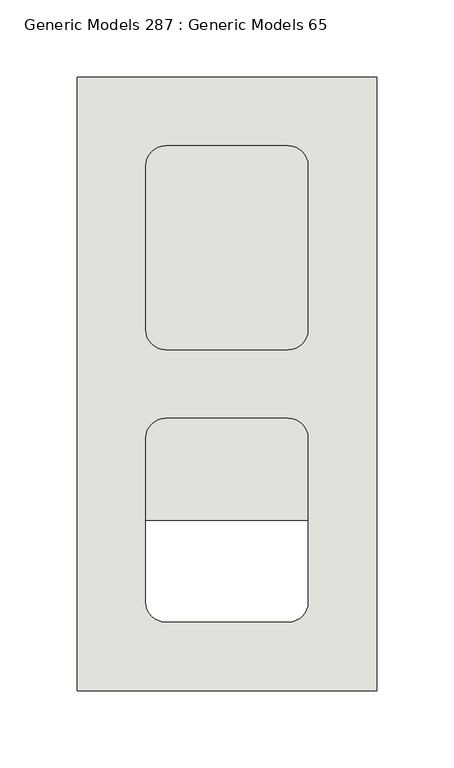
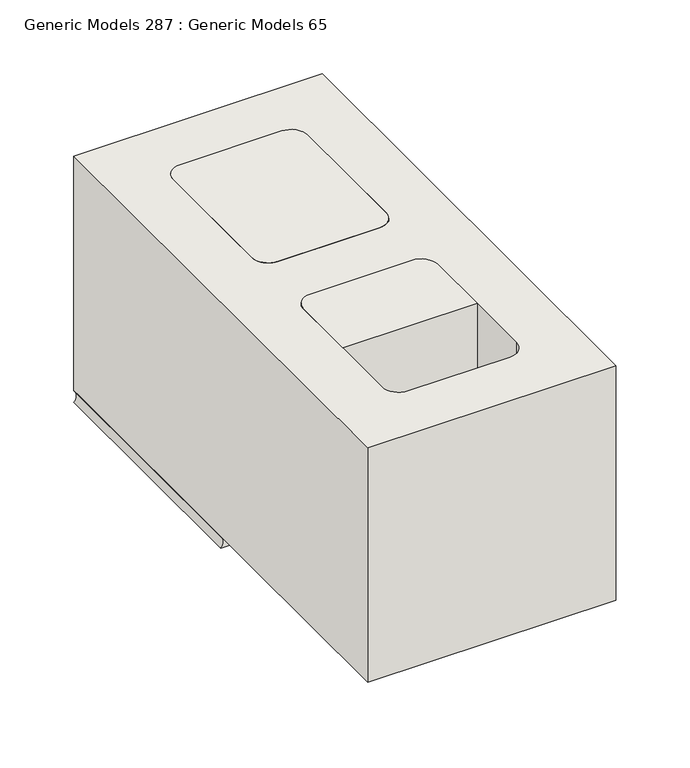
"""IFC4 building model written with IfcOpenShell, lengths in millimetres: wall geometry, Generic Models 287 : Generic Models 65."""

import ifcopenshell
import ifcopenshell.guid

model = None  # the IFC model being written
_history = None  # IfcOwnerHistory: only IFC2X3 demands one
_inside = {}  # id of a spatial element -> (the spatial element, [elements in it])
_under = {}  # id of a project, library or spatial element -> (it, [spatial elements below it])
_declared = {}  # id of a project -> (the project, [libraries it declares])
_typed = {}  # id of a type object -> (the type object, [elements of that type])
_made_of = {}  # id of a material, layer set ... -> (it, [elements and type objects made of it])


def new_model(schema):
    """Start an empty IFC model of exactly this schema.

    Asked for "IFC4X3", IfcOpenShell would pick the latest addendum, in which some entities
    have other attributes; the version numbers below select the first issue.
    IFC2X3 requires an IfcOwnerHistory on every rooted entity: one is made here for all.
    """
    global model, _history
    if schema == "IFC4X3":
        model = ifcopenshell.file(schema_version=(4, 3, 0, 0))
    else:
        model = ifcopenshell.file(schema=schema)
    _inside.clear()
    _under.clear()
    _declared.clear()
    _typed.clear()
    _made_of.clear()
    _history = None
    if model.schema == "IFC2X3":
        org = make("IfcOrganization", Name="unknown")
        user = make(
            "IfcPersonAndOrganization",
            ThePerson=make("IfcPerson", FamilyName="unknown"),
            TheOrganization=org,
        )
        app = make(
            "IfcApplication",
            ApplicationDeveloper=org,
            Version="unknown",
            ApplicationFullName="unknown",
            ApplicationIdentifier="unknown",
        )
        _history = make(
            "IfcOwnerHistory",
            OwningUser=user,
            OwningApplication=app,
            ChangeAction="ADDED",
            CreationDate=0,
        )
    return model


def make(cls, **values):
    """One entity of the class cls with the attributes given. An attribute that is None is left unset."""
    return model.create_entity(
        cls, **{name: value for name, value in values.items() if value is not None}
    )


def rooted(cls, **values):
    """An entity with a GlobalId (a new one), such as an element, a storey or a relation."""
    return make(cls, GlobalId=ifcopenshell.guid.new(), OwnerHistory=_history, **values)


def si_unit(unit_type, name, prefix=None):
    """IfcSIUnit, for example si_unit("LENGTHUNIT", "METRE", prefix="MILLI")."""
    return make("IfcSIUnit", UnitType=unit_type, Prefix=prefix, Name=name)


def assignment(units):
    """IfcUnitAssignment: the units of a project."""
    return None if units is None else make("IfcUnitAssignment", Units=units)


def point(xyz):
    """IfcCartesianPoint."""
    return None if xyz is None else make("IfcCartesianPoint", Coordinates=xyz)


def direction(xyz):
    """IfcDirection."""
    return None if xyz is None else make("IfcDirection", DirectionRatios=xyz)


def frame(location, z_axis=None, x_axis=None):
    """IfcAxis2Placement3D, a coordinate frame: its origin and axes. An axis left out is left unset."""
    return make(
        "IfcAxis2Placement3D",
        Location=point(location),
        Axis=direction(z_axis),
        RefDirection=direction(x_axis),
    )


def frame_2d(location, x_axis=None):
    """IfcAxis2Placement2D, a coordinate frame in the plane: its origin and x axis."""
    return make(
        "IfcAxis2Placement2D", Location=point(location), RefDirection=direction(x_axis)
    )


def origin():
    """The frame at (0, 0, 0) with its axes left unset."""
    return frame((0.0, 0.0, 0.0))


def origin_with_axes():
    """The frame at (0, 0, 0) with the z axis (0, 0, 1) and the x axis (1, 0, 0) written out."""
    return frame((0.0, 0.0, 0.0), z_axis=(0.0, 0.0, 1.0), x_axis=(1.0, 0.0, 0.0))


def place(relative_to, where):
    """IfcLocalPlacement: puts the frame where relative to a parent placement (None: the world)."""
    return make(
        "IfcLocalPlacement", PlacementRelTo=relative_to, RelativePlacement=where
    )


def context(
    kind, dimensions, precision=None, world=None, true_north=None, identifier=None
):
    """IfcGeometricRepresentationContext, for example the 3D "Model" context."""
    return make(
        "IfcGeometricRepresentationContext",
        ContextIdentifier=identifier,
        ContextType=kind,
        CoordinateSpaceDimension=dimensions,
        Precision=precision,
        WorldCoordinateSystem=world,
        TrueNorth=true_north,
    )


def project(units=None, contexts=None):
    """IfcProject with its units and contexts."""
    return rooted(
        "IfcProject",
        Name="project",
        RepresentationContexts=contexts,
        UnitsInContext=assignment(units),
    )


def spatial(cls, under=None, at=None, **own):
    """A site, building, storey or space (cls), placed at a placement, below another one or the project."""
    s = rooted(cls, ObjectPlacement=at, **own)
    if under is not None:
        _under.setdefault(under.id(), (under, []))[1].append(s)
    return s


def polyline(points):
    """IfcPolyline through the points."""
    return make("IfcPolyline", Points=[point(p) for p in points])


def circle_curve(where, radius):
    """IfcCircle in the frame where."""
    return make("IfcCircle", Position=where, Radius=radius)


def trimmed(basis, trim1, trim2, sense, master):
    """IfcTrimmedCurve: the piece of a basis curve between two trims."""
    return make(
        "IfcTrimmedCurve",
        BasisCurve=basis,
        Trim1=trim1,
        Trim2=trim2,
        SenseAgreement=sense,
        MasterRepresentation=master,
    )


def segment(curve, same_sense, transition):
    """IfcCompositeCurveSegment."""
    return make(
        "IfcCompositeCurveSegment",
        Transition=transition,
        SameSense=same_sense,
        ParentCurve=curve,
    )


def composite_curve(segments, self_intersect=None):
    """IfcCompositeCurve: segments joined end to end."""
    return make("IfcCompositeCurve", Segments=segments, SelfIntersect=self_intersect)


def outline(outer, holes=None, kind="AREA"):
    """IfcArbitraryClosedProfileDef: a profile drawn as a closed curve; with holes, ...WithVoids."""
    if holes is None:
        return make("IfcArbitraryClosedProfileDef", ProfileType=kind, OuterCurve=outer)
    return make(
        "IfcArbitraryProfileDefWithVoids",
        ProfileType=kind,
        OuterCurve=outer,
        InnerCurves=holes,
    )


def extrude(swept, where, along, depth):
    """IfcExtrudedAreaSolid: the profile swept, set in the frame where, extruded along a direction by depth."""
    return make(
        "IfcExtrudedAreaSolid",
        SweptArea=swept,
        Position=where,
        ExtrudedDirection=direction(along),
        Depth=depth,
    )


def shape(context_of_items, identifier, shape_type, items):
    """IfcShapeRepresentation: the items that make up one representation, for example the "Body"."""
    return make(
        "IfcShapeRepresentation",
        ContextOfItems=context_of_items,
        RepresentationIdentifier=identifier,
        RepresentationType=shape_type,
        Items=items,
    )


def source(mapping_origin, context_of_items, identifier, shape_type, items):
    """IfcRepresentationMap: a shape defined once, which mapped items show again and again."""
    return make(
        "IfcRepresentationMap",
        MappingOrigin=mapping_origin,
        MappedRepresentation=shape(context_of_items, identifier, shape_type, items),
    )


def transform(
    local_origin,
    x_axis=None,
    y_axis=None,
    z_axis=None,
    scale=None,
    scale2=None,
    scale3=None,
    uniform=True,
):
    """IfcCartesianTransformationOperator3D, or its non-uniform kind. x_axis, y_axis, z_axis: its Axis1, 2, 3."""
    if uniform:
        return make(
            "IfcCartesianTransformationOperator3D",
            Axis1=direction(x_axis),
            Axis2=direction(y_axis),
            LocalOrigin=point(local_origin),
            Scale=scale,
            Axis3=direction(z_axis),
        )
    return make(
        "IfcCartesianTransformationOperator3DnonUniform",
        Axis1=direction(x_axis),
        Axis2=direction(y_axis),
        LocalOrigin=point(local_origin),
        Scale=scale,
        Axis3=direction(z_axis),
        Scale2=scale2,
        Scale3=scale3,
    )


def mapped(mapping_source, mapping_target):
    """IfcMappedItem: shows the shape of a source again, moved by a transform."""
    return make(
        "IfcMappedItem", MappingSource=mapping_source, MappingTarget=mapping_target
    )


def made_of(thing, what):
    """Note that an element or type object is made of a material, layer set ...; save() writes the relation."""
    if what is not None:
        _made_of.setdefault(what.id(), (what, []))[1].append(thing)
    return thing


def element(
    cls,
    number,
    at=None,
    inside=None,
    cuts=None,
    type_object=None,
    material=None,
    context=None,
    identifier="Body",
    shape_type=None,
    held_by="IfcProductDefinitionShape",
    body=None,
    shapes=None,
    **own,
):
    """One element of the class cls, such as IfcWall. Its Tag is "e" and its number.

    at: its placement. inside: the storey or other place that contains it. cuts: it is an
    opening in that element (IfcRelVoidsElement). A single representation is given by context,
    identifier, shape_type and body (its items); several are given by shapes. held_by: the class
    of the entity that holds the representations. save() writes the other relations.
    """
    e = rooted(cls, Tag="e%d" % number, ObjectPlacement=at, **own)
    if body is not None:
        shapes = [shape(context, identifier, shape_type, body)]
    if shapes is not None:
        e.Representation = make(held_by, Representations=shapes)
    if inside is not None:
        _inside.setdefault(inside.id(), (inside, []))[1].append(e)
    if cuts is not None:
        rooted(
            "IfcRelVoidsElement", RelatingBuildingElement=cuts, RelatedOpeningElement=e
        )
    if type_object is not None:
        _typed.setdefault(type_object.id(), (type_object, []))[1].append(e)
    return made_of(e, material)


def aggregate(whole, parts):
    """IfcRelAggregates: a whole, such as a stair, and the parts it consists of."""
    return rooted("IfcRelAggregates", RelatingObject=whole, RelatedObjects=parts)


def save(model, path):
    """Write the relations noted so far, then the file.

    IfcRelAggregates (storeys below a building ...), IfcRelContainedInSpatialStructure (elements
    in a storey), IfcRelDefinesByType, IfcRelAssociatesMaterial and IfcRelDeclares: one each for
    every whole, place, type object, material and project.
    """
    for whole, parts in _under.values():
        aggregate(whole, parts)
    for where, things in _inside.values():
        rooted(
            "IfcRelContainedInSpatialStructure",
            RelatedElements=things,
            RelatingStructure=where,
        )
    for kind, things in _typed.values():
        rooted("IfcRelDefinesByType", RelatedObjects=things, RelatingType=kind)
    for what, things in _made_of.values():
        rooted("IfcRelAssociatesMaterial", RelatedObjects=things, RelatingMaterial=what)
    for by, libraries in _declared.values():
        rooted("IfcRelDeclares", RelatingContext=by, RelatedDefinitions=libraries)
    model.write(path)


def plane_surface(at):
    """IfcPlane: the flat surface through the origin of the frame at, square to its z axis."""
    return make("IfcPlane", Position=at)


def revolved_surface(curve, axis_point, axis_direction):
    """IfcSurfaceOfRevolution: the curve turned about the line through axis_point along axis_direction."""
    return make(
        "IfcSurfaceOfRevolution",
        SweptCurve=make("IfcArbitraryOpenProfileDef", ProfileType="CURVE", Curve=curve),
        AxisPosition=make("IfcAxis1Placement", Location=point(axis_point), Axis=direction(axis_direction)),
    )


def advanced_brep(points, edges, surfaces, faces):
    """IfcAdvancedBrep: a solid bounded by faces that lie on surfaces and meet in shared edges.

    An edge is (start, end): straight between two places in points (the first is 0);
    or (start, end, curve); or (start, end, curve, False) where it runs against its curve.
    A face is (place in surfaces, loops), or (place, loops, False) where it looks against
    its surface's normal. A loop lists edges by number (the first is 1), with a minus sign
    where the edge is run from its end to its start. The first loop is the outer one.
    """
    corners = [point(p) for p in points]
    vertices = [make("IfcVertexPoint", VertexGeometry=c) for c in corners]
    made = []
    for start, end, *more in edges:
        made.append(
            make(
                "IfcEdgeCurve",
                EdgeStart=vertices[start],
                EdgeEnd=vertices[end],
                EdgeGeometry=more[0] if more else make("IfcPolyline", Points=[corners[start], corners[end]]),
                SameSense=more[1] if len(more) > 1 else True,
            )
        )
    hull = []
    for where, loops, *sense in faces:
        bounds = []
        for j, loop in enumerate(loops):
            ring = [make("IfcOrientedEdge", EdgeElement=made[abs(k) - 1], Orientation=k > 0) for k in loop]
            bounds.append(
                make(
                    "IfcFaceOuterBound" if j == 0 else "IfcFaceBound",
                    Bound=make("IfcEdgeLoop", EdgeList=ring),
                    Orientation=True,
                )
            )
        hull.append(make("IfcAdvancedFace", Bounds=bounds, FaceSurface=surfaces[where], SameSense=sense[0] if sense else True))
    return make("IfcAdvancedBrep", Outer=make("IfcClosedShell", CfsFaces=hull))


def generic_models_287_generic_models_65_ef469ebf(model_context):
    return source(origin(), model_context, "Body", "SolidModel", [
        advanced_brep(
        [(430198.2125, 503.2375, 9.525), (430004.5375, 503.2375, 9.525), (430004.5375, 503.2375, 0.0), (430198.2125, 503.2375, 0.0), (430198.2125, 701.675, 9.525), (430198.2125, 701.675, 0.0), (430004.5375, 701.675, 0.0), (430004.5375, 701.675, 9.525), (430153.7625, 538.1625, 9.525), (430141.0625, 525.4625, 9.525), (430061.6875, 525.4625, 9.525), (430048.9875, 538.1625, 9.525), (430048.9875, 644.525, 9.525), (430061.6875, 657.225, 9.525), (430141.0625, 657.225, 9.525), (430153.7625, 644.525, 9.525), (430141.0625, 525.4625, 0.0), (430153.7625, 538.1625, 0.0), (430061.6875, 525.4625, 0.0), (430048.9875, 538.1625, 0.0), (430048.9875, 644.525, 0.0), (430061.6875, 657.225, 0.0), (430141.0625, 657.225, 0.0), (430153.7625, 644.525, 0.0)],
        [
            (0, 1),
            (1, 2, circle_curve(frame((429999.6545028, 503.2375, 4.7625), z_axis=(0.0, 1.0, 0.0), x_axis=(1.0, 0.0, 0.0)), 6.8209287)),
            (2, 3),
            (3, 0, circle_curve(frame((430203.0954972, 503.2375, 4.7625), z_axis=(0.0, 1.0, 0.0), x_axis=(-1.0, 0.0, 0.0)), 6.8209287)),
            (4, 5, circle_curve(frame((430203.0954972, 701.675, 4.7625), z_axis=(0.0, -1.0, 0.0), x_axis=(-1.0, 0.0, 0.0)), 6.8209287)),
            (5, 6),
            (6, 7, circle_curve(frame((429999.6545028, 701.675, 4.7625), z_axis=(0.0, -1.0, 0.0), x_axis=(1.0, 0.0, 0.0)), 6.8209287)),
            (7, 4),
            (0, 4),
            (7, 1),
            (8, 9, circle_curve(frame((430141.0625, 538.1625, 9.525), z_axis=(0.0, 0.0, -1.0), x_axis=(-1.0, 0.0, 0.0)), 12.7)),
            (9, 10),
            (10, 11, circle_curve(frame((430061.6875, 538.1625, 9.525), z_axis=(0.0, 0.0, -1.0), x_axis=(-1.0, 0.0, 0.0)), 12.7)),
            (11, 12),
            (12, 13, circle_curve(frame((430061.6875, 644.525, 9.525), z_axis=(0.0, 0.0, -1.0), x_axis=(-1.0, 0.0, 0.0)), 12.7)),
            (13, 14),
            (14, 15, circle_curve(frame((430141.0625, 644.525, 9.525), z_axis=(0.0, 0.0, -1.0), x_axis=(-1.0, 0.0, 0.0)), 12.7)),
            (15, 8),
            (16, 9),
            (8, 17),
            (17, 16, circle_curve(frame((430141.0625, 538.1625, 0.0), z_axis=(0.0, 0.0, -1.0), x_axis=(-1.0, 0.0, 0.0)), 12.7)),
            (16, 18),
            (18, 10),
            (18, 19, circle_curve(frame((430061.6875, 538.1625, 0.0), z_axis=(0.0, 0.0, -1.0), x_axis=(-1.0, 0.0, 0.0)), 12.7)),
            (19, 11),
            (19, 20),
            (20, 12),
            (20, 21, circle_curve(frame((430061.6875, 644.525, 0.0), z_axis=(0.0, 0.0, -1.0), x_axis=(-1.0, 0.0, 0.0)), 12.7)),
            (21, 13),
            (21, 22),
            (22, 14),
            (22, 23, circle_curve(frame((430141.0625, 644.525, 0.0), z_axis=(0.0, 0.0, -1.0), x_axis=(-1.0, 0.0, 0.0)), 12.7)),
            (23, 15),
            (23, 17),
            (6, 2),
            (5, 3),
        ],
        [
            plane_surface(frame((430101.375, 503.2375, 9.921875), z_axis=(0.0, -1.0, 0.0), x_axis=(0.0, 0.0, 1.0))),
            plane_surface(frame((430101.375, 701.675, 9.921875), z_axis=(0.0, 1.0, 0.0), x_axis=(0.0, 0.0, 1.0))),
            plane_surface(frame((430198.2125, 503.2375, 9.525), z_axis=(0.0, 0.0, 1.0), x_axis=(0.0, 1.0, 0.0))),
            revolved_surface(polyline([(430128.3625, 538.1625, 9.525000000000006), (430128.3625, 538.1625, 0.0)]), (430141.0625, 538.1625, 193.675), (0.0, 0.0, 1.0)),
            plane_surface(frame((430061.6875, 525.4625, 193.675), z_axis=(0.0, 1.0, 0.0), x_axis=(0.0, 0.0, -1.0))),
            revolved_surface(polyline([(430048.9875, 538.1625, 9.525000000000006), (430048.9875, 538.1625, 0.0)]), (430061.6875, 538.1625, 193.675), (0.0, 0.0, 1.0)),
            plane_surface(frame((430048.9875, 644.525, 193.675), z_axis=(1.0, 0.0, 0.0), x_axis=(0.0, 0.0, -1.0))),
            revolved_surface(polyline([(430048.9875, 644.525, 9.525000000000006), (430048.9875, 644.525, 0.0)]), (430061.6875, 644.525, 193.675), (0.0, 0.0, 1.0)),
            plane_surface(frame((430141.0625, 657.225, 193.675), z_axis=(0.0, -1.0, 0.0), x_axis=(0.0, 0.0, -1.0))),
            revolved_surface(polyline([(430128.3625, 644.525, 9.525000000000006), (430128.3625, 644.525, 0.0)]), (430141.0625, 644.525, 193.675), (0.0, 0.0, 1.0)),
            plane_surface(frame((430153.7625, 538.1625, 193.675), z_axis=(-1.0, 0.0, 0.0), x_axis=(0.0, 0.0, -1.0))),
            revolved_surface(polyline([(430006.4754315, 701.675, 4.7625), (430006.4754315, 503.2375, 4.7625)]), (429999.6545028, 503.2375, 4.7625), (0.0, 1.0, 0.0)),
            plane_surface(frame((430004.5375, 503.2375, 0.0), z_axis=(0.0, 0.0, -1.0), x_axis=(0.0, 1.0, 0.0))),
            revolved_surface(polyline([(430196.2745685, 701.675, 4.7625), (430196.2745685, 503.2375, 4.7625)]), (430203.0954972, 503.2375, 4.7625), (0.0, 1.0, 0.0)),
        ],
        [
            (0, [[1, 2, 3, 4]]),
            (1, [[5, 6, 7, 8]]),
            (2, [[-1, 9, -8, 10], [11, 12, 13, 14, 15, 16, 17, 18]]),
            (3, [[19, -11, 20, 21]]),
            (4, [[-19, 22, 23, -12]]),
            (5, [[-23, 24, 25, -13]]),
            (6, [[-25, 26, 27, -14]]),
            (7, [[-27, 28, 29, -15]]),
            (8, [[-29, 30, 31, -16]]),
            (9, [[-31, 32, 33, -17]]),
            (10, [[-33, 34, -20, -18]]),
            (11, [[-2, -10, -7, 35]]),
            (12, [[-3, -35, -6, 36], [-21, -34, -32, -30, -28, -26, -24, -22]]),
            (13, [[-4, -36, -5, -9]]),
        ],
    ),
        extrude(outline(composite_curve([segment(trimmed(circle_curve(frame_2d((430141.0625, 538.1625)), 12.7), [point((430153.7625, 538.1625))], [point((430141.0625, 525.4625))], False, "CARTESIAN"), True, "CONTINUOUS"), segment(polyline([(430141.0625, 525.4625), (430061.6875, 525.4625)]), True, "CONTINUOUS"), segment(trimmed(circle_curve(frame_2d((430061.6875, 538.1625)), 12.7), [point((430061.6875, 525.4625))], [point((430048.9875, 538.1625))], False, "CARTESIAN"), True, "CONTINUOUS"), segment(polyline([(430048.9875, 538.1625), (430048.9875, 644.525)]), True, "CONTINUOUS"), segment(trimmed(circle_curve(frame_2d((430061.6875, 644.525)), 12.7), [point((430048.9875, 644.525))], [point((430061.6875, 657.225))], False, "CARTESIAN"), True, "CONTINUOUS"), segment(polyline([(430061.6875, 657.225), (430141.0625, 657.225)]), True, "CONTINUOUS"), segment(trimmed(circle_curve(frame_2d((430141.0625, 644.525)), 12.7), [point((430141.0625, 657.225))], [point((430153.7625, 644.525))], False, "CARTESIAN"), True, "CONTINUOUS"), segment(polyline([(430153.7625, 644.525), (430153.7625, 538.1625)]), True, "CONTINUOUS")], self_intersect=False)), origin_with_axes(), (0.0, 0.0, 1.0), 203.2),
        extrude(outline(composite_curve([segment(trimmed(circle_curve(frame_2d((430061.6875, 468.3125)), 12.7), [point((430048.9875, 468.3125))], [point((430061.6875, 481.0125))], False, "CARTESIAN"), True, "CONTINUOUS"), segment(polyline([(430061.6875, 481.0125), (430141.0625, 481.0125)]), True, "CONTINUOUS"), segment(trimmed(circle_curve(frame_2d((430141.0625, 468.3125)), 12.7), [point((430141.0625, 481.0125))], [point((430153.7625, 468.3125))], False, "CARTESIAN"), True, "CONTINUOUS"), segment(polyline([(430153.7625, 468.3125), (430153.7625, 415.13125), (430048.9875, 415.13125), (430048.9875, 468.3125)]), True, "CONTINUOUS")], self_intersect=False)), origin_with_axes(), (0.0, 0.0, 1.0), 203.2),
        extrude(outline(polyline([(430198.2125, 304.8), (430004.5375, 304.8), (430004.5375, 701.675), (430198.2125, 701.675), (430198.2125, 304.8)]), holes=[composite_curve([segment(polyline([(430153.7625, 538.1625), (430153.7625, 644.525)]), True, "CONTINUOUS"), segment(trimmed(circle_curve(frame_2d((430141.0625, 644.525)), 12.7), [point((430153.7625, 644.525))], [point((430141.0625, 657.225))], True, "CARTESIAN"), True, "CONTINUOUS"), segment(polyline([(430141.0625, 657.225), (430061.6875, 657.225)]), True, "CONTINUOUS"), segment(trimmed(circle_curve(frame_2d((430061.6875, 644.525)), 12.7), [point((430061.6875, 657.225))], [point((430048.9875, 644.525))], True, "CARTESIAN"), True, "CONTINUOUS"), segment(polyline([(430048.9875, 644.525), (430048.9875, 538.1625)]), True, "CONTINUOUS"), segment(trimmed(circle_curve(frame_2d((430061.6875, 538.1625)), 12.7), [point((430048.9875, 538.1625))], [point((430061.6875, 525.4625))], True, "CARTESIAN"), True, "CONTINUOUS"), segment(polyline([(430061.6875, 525.4625), (430141.0625, 525.4625)]), True, "CONTINUOUS"), segment(trimmed(circle_curve(frame_2d((430141.0625, 538.1625)), 12.7), [point((430141.0625, 525.4625))], [point((430153.7625, 538.1625))], True, "CARTESIAN"), True, "CONTINUOUS")], self_intersect=False), composite_curve([segment(polyline([(430048.9875, 468.3125), (430048.9875, 361.95)]), True, "CONTINUOUS"), segment(trimmed(circle_curve(frame_2d((430061.6875, 361.95)), 12.7), [point((430048.9875, 361.95))], [point((430061.6875, 349.25))], True, "CARTESIAN"), True, "CONTINUOUS"), segment(polyline([(430061.6875, 349.25), (430141.0625, 349.25)]), True, "CONTINUOUS"), segment(trimmed(circle_curve(frame_2d((430141.0625, 361.95)), 12.7), [point((430141.0625, 349.25))], [point((430153.7625, 361.95))], True, "CARTESIAN"), True, "CONTINUOUS"), segment(polyline([(430153.7625, 361.95), (430153.7625, 468.3125)]), True, "CONTINUOUS"), segment(trimmed(circle_curve(frame_2d((430141.0625, 468.3125)), 12.7), [point((430153.7625, 468.3125))], [point((430141.0625, 481.0125))], True, "CARTESIAN"), True, "CONTINUOUS"), segment(polyline([(430141.0625, 481.0125), (430061.6875, 481.0125)]), True, "CONTINUOUS"), segment(trimmed(circle_curve(frame_2d((430061.6875, 468.3125)), 12.7), [point((430061.6875, 481.0125))], [point((430048.9875, 468.3125))], True, "CARTESIAN"), True, "CONTINUOUS")], self_intersect=False)]), frame((0.0, 0.0, 9.525), z_axis=(0.0, 0.0, 1.0), x_axis=(1.0, 0.0, 0.0)), (0.0, 0.0, 1.0), 193.675),
    ])


if __name__ == "__main__":
    model = new_model("IFC4")
    model_context = context("Model", 3, world=origin())
    ifc_project = project(units=[si_unit("LENGTHUNIT", "METRE", prefix="MILLI")], contexts=[model_context])
    site = spatial("IfcSite", under=ifc_project)
    building = spatial("IfcBuilding", under=site)
    placement = place(None, origin())
    generic_models_287_generic_models_65_shape = generic_models_287_generic_models_65_ef469ebf(model_context)
    element("IfcWall", 1, ObjectType="Generic Models 287 : Generic Models 65", at=placement, inside=building, context=model_context, shape_type="MappedRepresentation", body=[
        mapped(generic_models_287_generic_models_65_shape, transform((0.0, 0.0, 0.0), x_axis=(1.0, 0.0, 0.0), y_axis=(0.0, 1.0, 0.0), z_axis=(0.0, 0.0, 1.0))),
    ])
    save(model, "model.ifc")

# Revit data of these elements
# Element 1 (IfcWall, "Generic Models 287 : Generic Models 65")
#   Materials on its faces: "CMU (SEE 'WALL TAG' FOR SIZE)", "FILL CORE IF APPLICABLE - SEE STRUCTURAL DWGS FOR DETAILS", "MORTAR JOINT"
# Materials
#   "CMU (SEE 'WALL TAG' FOR SIZE)": class "Masonry", colour RGB 203 203 199, transparency 0, Description = "Concrete masonry units", Cost = 0
#   "FILL CORE IF APPLICABLE - SEE STRUCTURAL DWGS FOR DETAILS": class "Generic", colour RGB 170 170 170, transparency 0, Cost = 0
#   "MORTAR JOINT": class "Generic", colour RGB 120 120 120, transparency 0, Cost = 0
